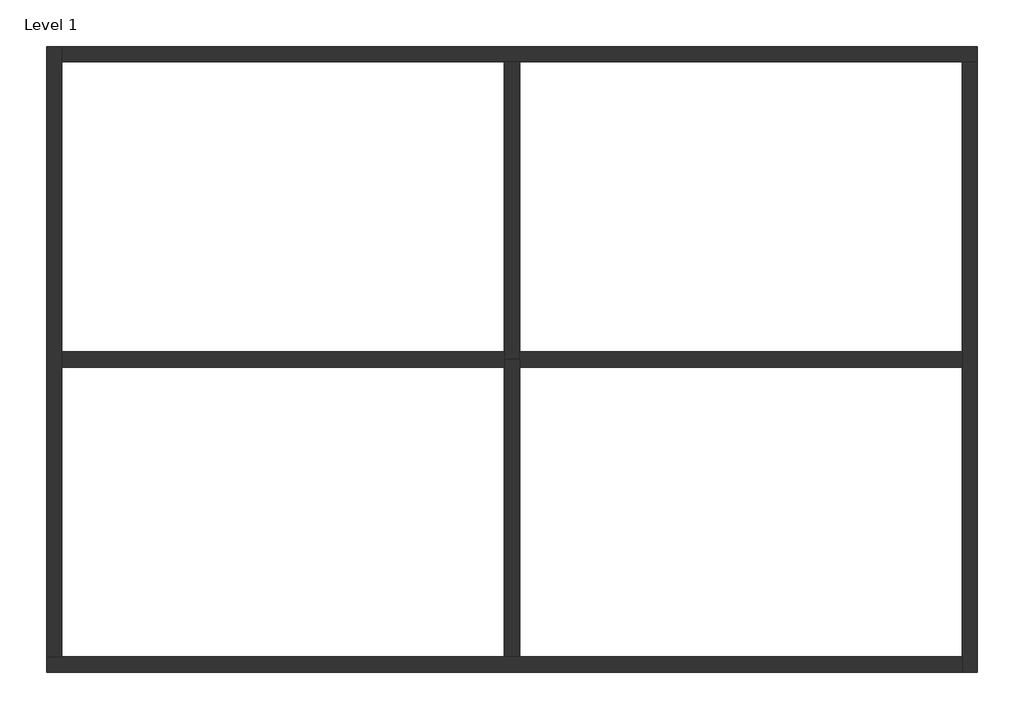
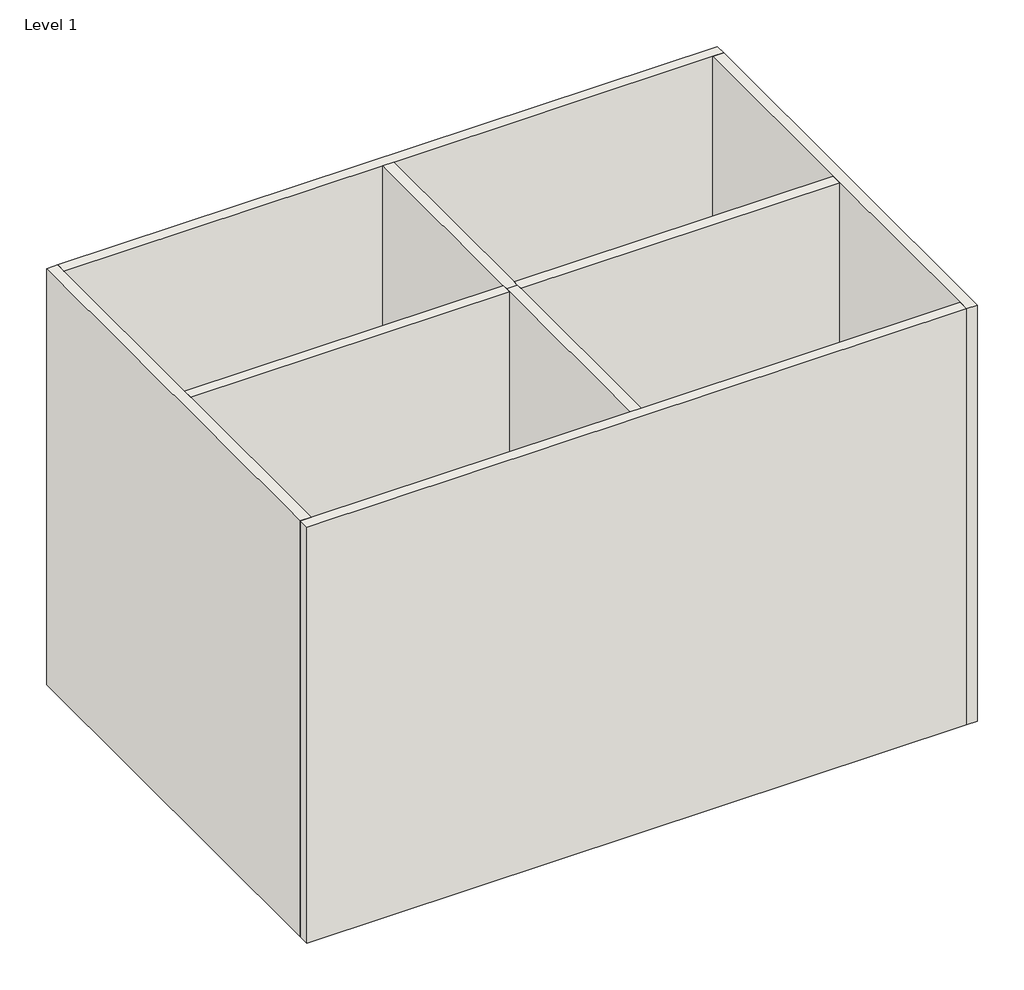
# One storey: 8 walls.
"""IFC4 building model written with IfcOpenShell, lengths in millimetres."""

from ifc_helpers import new_model, si_unit, origin, place, context, project, spatial, faceted_brep, element, save

model = new_model("IFC4")

# Units and contexts
model_context = context("Model", 3, world=origin())
ifc_project = project(units=[si_unit("LENGTHUNIT", "METRE", prefix="MILLI")], contexts=[model_context])

# Site, building, storey
site = spatial("IfcSite", under=ifc_project)
building = spatial("IfcBuilding", under=site)
storey = spatial("IfcBuildingStorey", under=building, Name="Level 1", Elevation=0.0)

# Walls
placement = place(None, origin())
element("IfcWall", 1, ObjectType="Generic - 6\"", at=placement, inside=storey, context=model_context, shape_type="Brep", body=[
    faceted_brep([(0.0, 0.0, 0.0), (9144.0, 0.0, 0.0), (9144.0, 0.0, 6096.0), (0.0, 0.0, 6096.0), (0.0, 152.4, 0.0), (0.0, 152.4, 6096.0), (152.4, 152.4, 6096.0), (4572.0, 152.4, 6096.0), (4724.4, 152.4, 6096.0), (9144.0, 152.4, 6096.0), (9144.0, 152.4, 0.0), (4724.4, 152.4, 0.0), (4572.0, 152.4, 0.0), (152.4, 152.4, 0.0)], [[[0, 1, 2, 3]], [[4, 5, 6, 7, 8, 9, 10, 11, 12, 13]], [[1, 0, 4, 13, 12, 11, 10]], [[3, 2, 9, 8, 7, 6, 5]], [[0, 3, 5, 4]], [[2, 1, 10, 9]]]),
])
element("IfcWall", 2, ObjectType="Generic - 6\"", at=placement, inside=storey, context=model_context, shape_type="Brep", body=[
    faceted_brep([(0.0, 6248.4, 0.0), (0.0, 152.4, 0.0), (0.0, 152.4, 6096.0), (0.0, 6248.4, 6096.0), (152.4, 6248.4, 0.0), (152.4, 6248.4, 6096.0), (152.4, 6096.0, 6096.0), (152.4, 3200.4, 6096.0), (152.4, 3048.0, 6096.0), (152.4, 152.4, 6096.0), (152.4, 152.4, 0.0), (152.4, 3048.0, 0.0), (152.4, 3200.4, 0.0), (152.4, 6096.0, 0.0)], [[[0, 1, 2, 3]], [[4, 5, 6, 7, 8, 9, 10, 11, 12, 13]], [[1, 0, 4, 13, 12, 11, 10]], [[3, 2, 9, 8, 7, 6, 5]], [[0, 3, 5, 4]], [[2, 1, 10, 9]]]),
])
element("IfcWall", 3, ObjectType="Generic - 6\"", at=placement, inside=storey, context=model_context, shape_type="Brep", body=[
    faceted_brep([(9296.4, 6248.4, 0.0), (152.4, 6248.4, 0.0), (152.4, 6248.4, 6096.0), (9296.4, 6248.4, 6096.0), (9296.4, 6096.0, 0.0), (9296.4, 6096.0, 6096.0), (9144.0, 6096.0, 6096.0), (4724.4, 6096.0, 6096.0), (4572.0, 6096.0, 6096.0), (152.4, 6096.0, 6096.0), (152.4, 6096.0, 0.0), (4572.0, 6096.0, 0.0), (4724.4, 6096.0, 0.0), (9144.0, 6096.0, 0.0)], [[[0, 1, 2, 3]], [[4, 5, 6, 7, 8, 9, 10, 11, 12, 13]], [[1, 0, 4, 13, 12, 11, 10]], [[3, 2, 9, 8, 7, 6, 5]], [[0, 3, 5, 4]], [[2, 1, 10, 9]]]),
])
element("IfcWall", 4, ObjectType="Generic - 6\"", at=placement, inside=storey, context=model_context, shape_type="Brep", body=[
    faceted_brep([(9296.4, 0.0, 0.0), (9296.4, 6096.0, 0.0), (9296.4, 6096.0, 6096.0), (9296.4, 0.0, 6096.0), (9144.0, 0.0, 0.0), (9144.0, 0.0, 6096.0), (9144.0, 152.4, 6096.0), (9144.0, 3048.0, 6096.0), (9144.0, 3200.4, 6096.0), (9144.0, 6096.0, 6096.0), (9144.0, 6096.0, 0.0), (9144.0, 3200.4, 0.0), (9144.0, 3048.0, 0.0), (9144.0, 152.4, 0.0)], [[[0, 1, 2, 3]], [[4, 5, 6, 7, 8, 9, 10, 11, 12, 13]], [[1, 0, 4, 13, 12, 11, 10]], [[3, 2, 9, 8, 7, 6, 5]], [[0, 3, 5, 4]], [[2, 1, 10, 9]]]),
])
element("IfcWall", 5, ObjectType="Generic - 6\"", at=placement, inside=storey, context=model_context, shape_type="Brep", body=[
    faceted_brep([(4572.0, 6096.0, 0.0), (4572.0, 3200.4, 0.0), (4572.0, 3124.2, 0.0), (4572.0, 3124.2, 6096.0), (4572.0, 3200.4, 6096.0), (4572.0, 6096.0, 6096.0), (4724.4, 6096.0, 0.0), (4724.4, 6096.0, 6096.0), (4724.4, 3200.4, 6096.0), (4724.4, 3124.2, 6096.0), (4724.4, 3124.2, 0.0), (4724.4, 3200.4, 0.0)], [[[0, 1, 2, 3, 4, 5]], [[6, 7, 8, 9, 10, 11]], [[2, 1, 0, 6, 11, 10]], [[3, 2, 10, 9]], [[5, 4, 3, 9, 8, 7]], [[0, 5, 7, 6]]]),
])
element("IfcWall", 6, ObjectType="Generic - 6\"", at=placement, inside=storey, context=model_context, shape_type="Brep", body=[
    faceted_brep([(9144.0, 3200.4, 0.0), (4724.4, 3200.4, 0.0), (4724.4, 3200.4, 6096.0), (9144.0, 3200.4, 6096.0), (9144.0, 3048.0, 0.0), (9144.0, 3048.0, 6096.0), (4724.4, 3048.0, 6096.0), (4724.4, 3048.0, 0.0), (4724.4, 3124.2, 0.0), (4724.4, 3124.2, 6096.0)], [[[0, 1, 2, 3]], [[4, 5, 6, 7]], [[1, 0, 4, 7, 8]], [[3, 2, 9, 6, 5]], [[0, 3, 5, 4]], [[2, 1, 8, 7, 6, 9]]]),
])
element("IfcWall", 7, ObjectType="Generic - 6\"", at=placement, inside=storey, context=model_context, shape_type="Brep", body=[
    faceted_brep([(4572.0, 3200.4, 0.0), (152.4, 3200.4, 0.0), (152.4, 3200.4, 6096.0), (4572.0, 3200.4, 6096.0), (4572.0, 3048.0, 0.0), (4572.0, 3048.0, 6096.0), (152.4, 3048.0, 6096.0), (152.4, 3048.0, 0.0), (4572.0, 3124.2, 0.0), (4572.0, 3124.2, 6096.0)], [[[0, 1, 2, 3]], [[4, 5, 6, 7]], [[1, 0, 8, 4, 7]], [[3, 2, 6, 5, 9]], [[2, 1, 7, 6]], [[0, 3, 9, 5, 4, 8]]]),
])
element("IfcWall", 8, ObjectType="Generic - 6\"", at=placement, inside=storey, context=model_context, shape_type="Brep", body=[
    faceted_brep([(4572.0, 3124.2, 0.0), (4572.0, 3048.0, 0.0), (4572.0, 152.4, 0.0), (4572.0, 152.4, 6096.0), (4572.0, 3048.0, 6096.0), (4572.0, 3124.2, 6096.0), (4724.4, 3124.2, 0.0), (4724.4, 3124.2, 6096.0), (4724.4, 3048.0, 6096.0), (4724.4, 152.4, 6096.0), (4724.4, 152.4, 0.0), (4724.4, 3048.0, 0.0)], [[[0, 1, 2, 3, 4, 5]], [[6, 7, 8, 9, 10, 11]], [[2, 1, 0, 6, 11, 10]], [[5, 4, 3, 9, 8, 7]], [[0, 5, 7, 6]], [[3, 2, 10, 9]]]),
])

save(model, "model.ifc")

# Revit data of these elements
# Project information
#   Project Issue Date = "Issue Date"
#   Project Status = "Project Status"
#   Client Name = "Owner"
#   Project Address = "Enter address here"
#   Project Name = "PROJECT NAME"
#   Project Number = "Project Number"
# Type "Generic - 6\""
#   Assembly Code = "B2010"
#   Width = 0' - 6"
#   Layers, outside or top first: 0' - 6" no material (function 1)
# Elements 1, 2, 3, 4 (IfcWall, "Generic - 6\"")
#   Top Offset = 0' - 0"
#   Base Offset = 0' - 0"
#   Unconnected Height = 20' - 0"
#   wall height = 20' - 0"
#   Phase Created = New Construction
#   Base Constraint = Level 1
#   Materials on its faces: "Default Wall"
# Element 5 (IfcWall, "Generic - 6\"")
#   OD_Option_2 = "N"
#   OD_Option_4 = "N"
#   Top Offset = 0' - 0"
#   Base Offset = 0' - 0"
#   Unconnected Height = 20' - 0"
#   wall height = 20' - 0"
#   Phase Created = New Construction
#   Base Constraint = Level 1
#   Materials on its faces: "Default Wall"
# Element 6 (IfcWall, "Generic - 6\"")
#   OD_Option_1 = ""
#   OD_Option_3 = "N"
#   OD_Option_4 = "N"
#   Top Offset = 0' - 0"
#   Base Offset = 0' - 0"
#   Unconnected Height = 20' - 0"
#   wall height = 20' - 0"
#   Phase Created = New Construction
#   Base Constraint = Level 1
#   Materials on its faces: "Default Wall"
# Element 7 (IfcWall, "Generic - 6\"")
#   OD_Option_3 = "N"
#   OD_Option_4 = "N"
#   Top Offset = 0' - 0"
#   Base Offset = 0' - 0"
#   Unconnected Height = 20' - 0"
#   wall height = 20' - 0"
#   Phase Created = New Construction
#   Base Constraint = Level 1
#   Materials on its faces: "Default Wall"
# Element 8 (IfcWall, "Generic - 6\"")
#   OD_Option_1 = ""
#   OD_Option_2 = "N"
#   OD_Option_4 = "N"
#   Top Offset = 0' - 0"
#   Base Offset = 0' - 0"
#   Unconnected Height = 20' - 0"
#   wall height = 20' - 0"
#   Phase Created = New Construction
#   Base Constraint = Level 1
#   Materials on its faces: "Default Wall"
# Materials
#   "Default Wall": class "Miscellaneous", colour RGB 80 80 80, transparency 0
